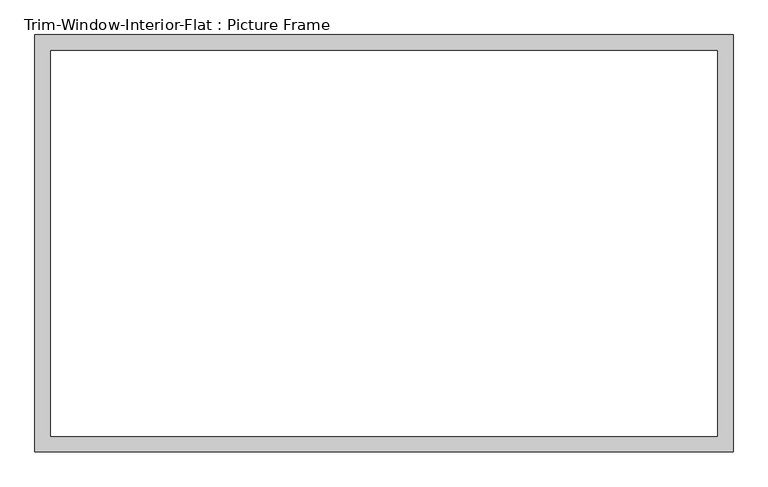
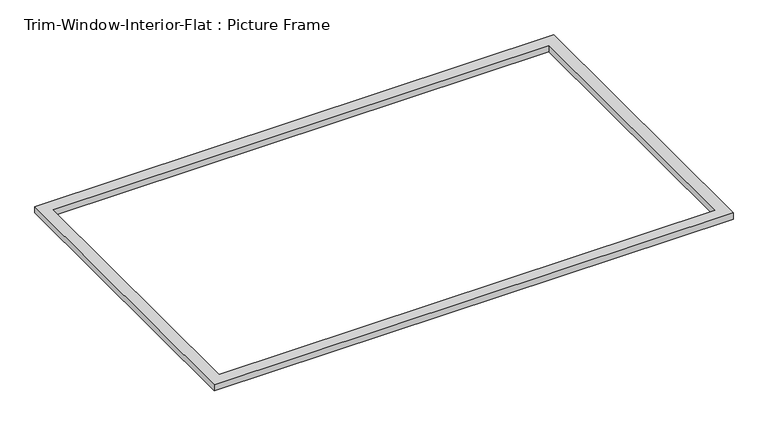
"""IFC4 building model written with IfcOpenShell, lengths in millimetres: proxy geometry, Trim-Window-Interior-Flat : Picture Frame."""

from ifc_helpers import new_model, si_unit, origin, origin_with_axes, place, context, project, spatial, polyline, outline, extrude, source, transform, mapped, element, save


def trim_window_interior_flat_picture_frame_b9a42e7f(model_context):
    return source(origin(), model_context, "Body", "SweptSolid", [
        extrude(outline(polyline([(1263.65, 44.45), (1263.65, -1466.85), (-1263.65, -1466.85), (-1263.65, 44.45), (1263.65, 44.45)]), holes=[polyline([(1206.5, -12.7), (-1206.5, -12.7), (-1206.5, -1409.7), (1206.5, -1409.7), (1206.5, -12.7)])]), origin_with_axes(), (0.0, 0.0, 1.0), 31.75),
    ])


if __name__ == "__main__":
    model = new_model("IFC4")
    model_context = context("Model", 3, world=origin())
    ifc_project = project(units=[si_unit("LENGTHUNIT", "METRE", prefix="MILLI")], contexts=[model_context])
    site = spatial("IfcSite", under=ifc_project)
    building = spatial("IfcBuilding", under=site)
    placement = place(None, origin())
    trim_window_interior_flat_picture_frame_shape = trim_window_interior_flat_picture_frame_b9a42e7f(model_context)
    element("IfcBuildingElementProxy", 1, Name="Trim-Window-Interior-Flat : Picture Frame", ObjectType="Trim-Window-Interior-Flat : Picture Frame", at=placement, inside=building, context=model_context, shape_type="MappedRepresentation", body=[
        mapped(trim_window_interior_flat_picture_frame_shape, transform((0.0, 0.0, 0.0), x_axis=(1.0, 0.0, 0.0), y_axis=(0.0, 1.0, 0.0), z_axis=(0.0, 0.0, 1.0))),
    ])
    save(model, "model.ifc")

# Revit data of these elements
# Type "Trim-Window-Interior-Flat : Picture Frame"
#   Trim Thickness_Picture Frame = 0' - 1 1/4"
#   Trim Width = 0' - 2 1/4"
#   Trim Thickness_with Sill = 0' - 0 3/4"
#   Sill Thickness = 0' - 1 1/4"
#   Opening Width [instance default] = 2' - 0"
#   Opening Height [instance default] = 3' - 0"
#   Default Elevation = 4' - 0"
#   Sill = no
#   Picture Frame = yes
#   Trim Material [instance default] = none
# Element 1 (IfcBuildingElementProxy, "Trim-Window-Interior-Flat : Picture Frame")
#   Opening Width = 8' - 0"
#   Opening Height = 4' - 8"
#   Trim Material = Wood - Stained
#   Materials on its faces: "Wood - Stained"
# Materials
#   "Wood - Stained": class "Wood", colour RGB 224 178 126, transparency 0, Cost = 0
